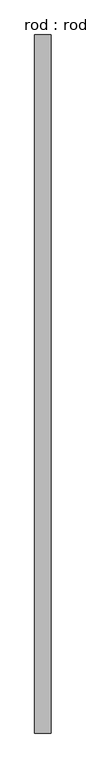
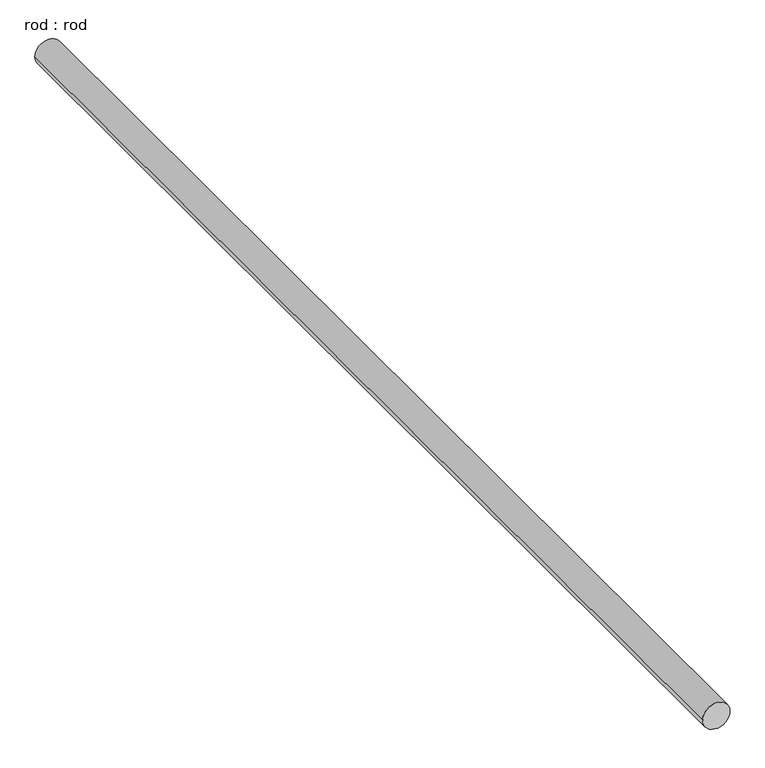
"""IFC4 building model written with IfcOpenShell, lengths in millimetres: proxy geometry, rod : rod."""

from ifc_helpers import new_model, si_unit, point, frame, frame_2d, origin, place, context, project, spatial, circle_curve, trimmed, segment, composite_curve, outline, extrude, source, transform, mapped, element, save


def rod_rod_a9224c9c(model_context):
    return source(origin(), model_context, "Body", "SweptSolid", [
        extrude(outline(composite_curve([segment(trimmed(circle_curve(frame_2d((0.0108462, 0.0)), 200.0), [point((0.0108462, 200.0))], [point((0.0108462, -200.0))], False, "CARTESIAN"), True, "CONTINUOUS"), segment(trimmed(circle_curve(frame_2d((0.0108462, 0.0)), 200.0), [point((0.0108462, -200.0))], [point((0.0108462, 200.0))], False, "CARTESIAN"), True, "CONTINUOUS")], self_intersect=False)), frame((0.0, -4398.5168763, 0.0), z_axis=(0.0, 1.0, 0.0), x_axis=(0.0, 0.0, 1.0)), (0.0, 0.0, 1.0), 16982.4909834),
    ])


if __name__ == "__main__":
    model = new_model("IFC4")
    model_context = context("Model", 3, world=origin())
    ifc_project = project(units=[si_unit("LENGTHUNIT", "METRE", prefix="MILLI")], contexts=[model_context])
    site = spatial("IfcSite", under=ifc_project)
    building = spatial("IfcBuilding", under=site)
    placement = place(None, origin())
    rod_rod_shape = rod_rod_a9224c9c(model_context)
    element("IfcBuildingElementProxy", 1, Name="rod : rod", ObjectType="rod : rod", at=placement, inside=building, context=model_context, shape_type="MappedRepresentation", body=[
        mapped(rod_rod_shape, transform((0.0, 0.0, 0.0), x_axis=(1.0, 0.0, 0.0), y_axis=(0.0, 1.0, 0.0), z_axis=(0.0, 0.0, 1.0))),
    ])
    save(model, "model.ifc")

# Revit data of these elements
# Type "rod : rod"
#   Default Elevation = 0
